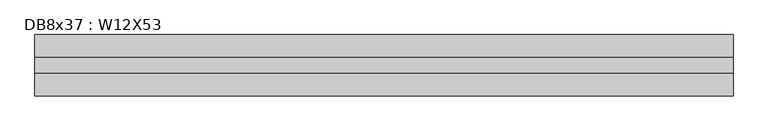
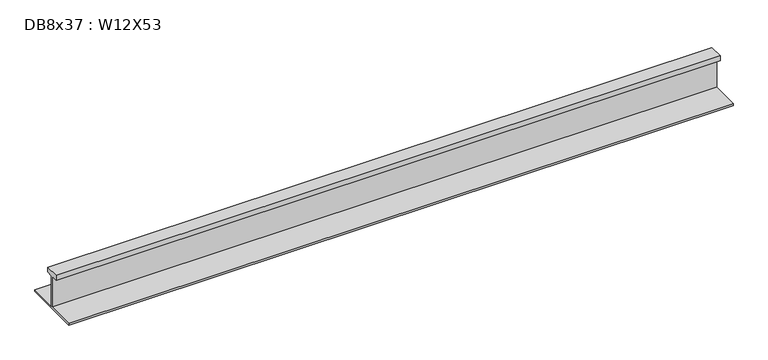
"""IFC4 building model written with IfcOpenShell, lengths in millimetres: beam geometry, DB8x37 : W12X53."""

from ifc_helpers import new_model, si_unit, frame, origin, place, context, project, spatial, polyline, outline, extrude, source, transform, mapped, element, save


def db8x37_w12x53_5b28efc3(model_context):
    return source(origin(), model_context, "Body", "SweptSolid", [
        extrude(outline(polyline([(38.1, 145.415), (38.1, 120.015), (2.921, 120.015), (2.921, -48.4505), (152.4, -48.4505), (152.4, -58.1025), (-152.4, -58.1025), (-152.4, -48.4505), (-2.921, -48.4505), (-2.921, 120.015), (-38.1, 120.015), (-38.1, 145.415), (38.1, 145.415)])), frame((-1724.7091296, 0.0, 0.0), z_axis=(1.0, 0.0, 0.0), x_axis=(0.0, 1.0, 0.0)), (0.0, 0.0, 1.0), 3456.8254171),
    ])


if __name__ == "__main__":
    model = new_model("IFC4")
    model_context = context("Model", 3, world=origin())
    ifc_project = project(units=[si_unit("LENGTHUNIT", "METRE", prefix="MILLI")], contexts=[model_context])
    site = spatial("IfcSite", under=ifc_project)
    building = spatial("IfcBuilding", under=site)
    placement = place(None, origin())
    db8x37_w12x53_shape = db8x37_w12x53_5b28efc3(model_context)
    element("IfcBeam", 1, ObjectType="DB8x37 : W12X53", at=placement, inside=building, context=model_context, shape_type="MappedRepresentation", body=[
        mapped(db8x37_w12x53_shape, transform((0.0, 0.0, 0.0), x_axis=(1.0, 0.0, 0.0), y_axis=(0.0, 1.0, 0.0), z_axis=(0.0, 0.0, 1.0))),
    ])
    save(model, "model.ifc")

# Revit data of these elements
# Type "DB8x37 : W12X53"
#   Assembly Code = "B10"
#   W = 53
#   Length [instance default] = 5' - 0"
#   bf = 0' - 10"
#   d = 1' - 0.1"
#   k = 0' - 1 3/8"
#   k2 = 0' - 0.8"
#   tf = 0' - 0.575"
#   tw = 0' - 0.345"
#   A = 0.108333 SF
#   Structural Material [instance default] = Steel ASTM A992
# Element 1 (IfcBeam, "DB8x37 : W12X53")
#   Materials on its faces: "Steel ASTM A992"
# Materials
#   "Steel ASTM A992": class "Metal", colour RGB 199 199 199, transparency 0, Description = "Structural steel 50ksi", Cost = 0
